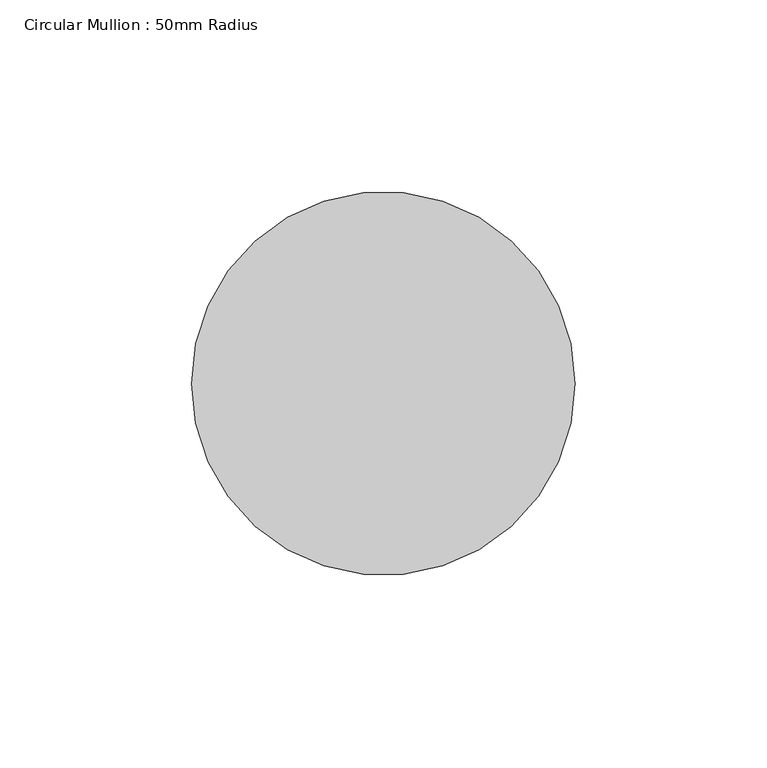
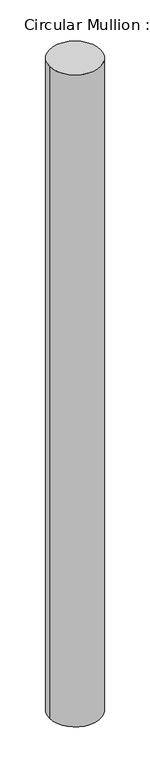
"""IFC4 building model written with IfcOpenShell, lengths in millimetres: member geometry, Circular Mullion : 50mm Radius."""

from ifc_helpers import new_model, si_unit, point, frame, origin, origin_2d, place, context, project, spatial, circle_curve, trimmed, segment, composite_curve, outline, extrude, source, transform, mapped, element, save


def circular_mullion_50mm_radius_65030307(model_context):
    return source(origin(), model_context, "Body", "SweptSolid", [
        extrude(outline(composite_curve([segment(trimmed(circle_curve(origin_2d(), 50.0), [point((50.0, 0.0))], [point((-50.0, 0.0))], False, "CARTESIAN"), True, "CONTINUOUS"), segment(trimmed(circle_curve(origin_2d(), 50.0), [point((-50.0, 0.0))], [point((50.0, 0.0))], False, "CARTESIAN"), True, "CONTINUOUS")], self_intersect=False)), frame((0.0, 0.0, -1349.8110202), z_axis=(0.0, 0.0, 1.0), x_axis=(1.0, 0.0, 0.0)), (0.0, 0.0, 1.0), 1349.8110202),
    ])


if __name__ == "__main__":
    model = new_model("IFC4")
    model_context = context("Model", 3, world=origin())
    ifc_project = project(units=[si_unit("LENGTHUNIT", "METRE", prefix="MILLI")], contexts=[model_context])
    site = spatial("IfcSite", under=ifc_project)
    building = spatial("IfcBuilding", under=site)
    placement = place(None, origin())
    circular_mullion_50mm_radius_shape = circular_mullion_50mm_radius_65030307(model_context)
    element("IfcMember", 1, ObjectType="Circular Mullion : 50mm Radius", at=placement, inside=building, context=model_context, shape_type="MappedRepresentation", body=[
        mapped(circular_mullion_50mm_radius_shape, transform((0.0, 0.0, 0.0), x_axis=(1.0, 0.0, 0.0), y_axis=(0.0, 1.0, 0.0), z_axis=(0.0, 0.0, 1.0))),
    ])
    save(model, "model.ifc")

# Revit data of these elements
# Type "Circular Mullion : 50mm Radius"
#   built-in parameter 1007350 = 0.164042 (stored number, unit not read)
# Element 1 (IfcMember, "Circular Mullion : 50mm Radius")
#   Materials on its faces: "Aluminium"
# Materials
#   "Aluminium": class "Metal", colour RGB 247 247 247, transparency 0, Description = "Aluminium 6061", Cost = 0
